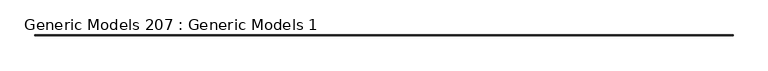
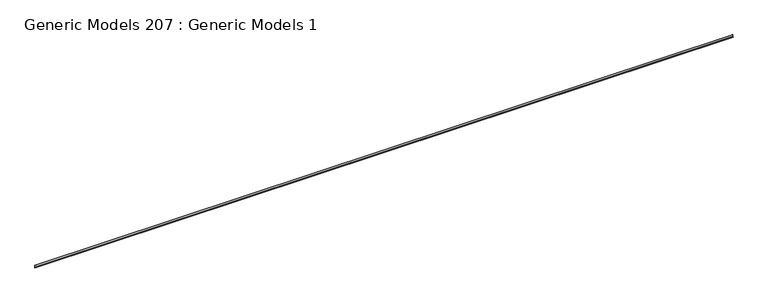
"""IFC4 building model written with IfcOpenShell, lengths in millimetres: proxy geometry, Generic Models 207 : Generic Models 1."""

import ifcopenshell
import ifcopenshell.guid

model = None  # the IFC model being written
_history = None  # IfcOwnerHistory: only IFC2X3 demands one
_inside = {}  # id of a spatial element -> (the spatial element, [elements in it])
_under = {}  # id of a project, library or spatial element -> (it, [spatial elements below it])
_declared = {}  # id of a project -> (the project, [libraries it declares])
_typed = {}  # id of a type object -> (the type object, [elements of that type])
_made_of = {}  # id of a material, layer set ... -> (it, [elements and type objects made of it])


def new_model(schema):
    """Start an empty IFC model of exactly this schema.

    Asked for "IFC4X3", IfcOpenShell would pick the latest addendum, in which some entities
    have other attributes; the version numbers below select the first issue.
    IFC2X3 requires an IfcOwnerHistory on every rooted entity: one is made here for all.
    """
    global model, _history
    if schema == "IFC4X3":
        model = ifcopenshell.file(schema_version=(4, 3, 0, 0))
    else:
        model = ifcopenshell.file(schema=schema)
    _inside.clear()
    _under.clear()
    _declared.clear()
    _typed.clear()
    _made_of.clear()
    _history = None
    if model.schema == "IFC2X3":
        org = make("IfcOrganization", Name="unknown")
        user = make(
            "IfcPersonAndOrganization",
            ThePerson=make("IfcPerson", FamilyName="unknown"),
            TheOrganization=org,
        )
        app = make(
            "IfcApplication",
            ApplicationDeveloper=org,
            Version="unknown",
            ApplicationFullName="unknown",
            ApplicationIdentifier="unknown",
        )
        _history = make(
            "IfcOwnerHistory",
            OwningUser=user,
            OwningApplication=app,
            ChangeAction="ADDED",
            CreationDate=0,
        )
    return model


def make(cls, **values):
    """One entity of the class cls with the attributes given. An attribute that is None is left unset."""
    return model.create_entity(
        cls, **{name: value for name, value in values.items() if value is not None}
    )


def rooted(cls, **values):
    """An entity with a GlobalId (a new one), such as an element, a storey or a relation."""
    return make(cls, GlobalId=ifcopenshell.guid.new(), OwnerHistory=_history, **values)


def si_unit(unit_type, name, prefix=None):
    """IfcSIUnit, for example si_unit("LENGTHUNIT", "METRE", prefix="MILLI")."""
    return make("IfcSIUnit", UnitType=unit_type, Prefix=prefix, Name=name)


def assignment(units):
    """IfcUnitAssignment: the units of a project."""
    return None if units is None else make("IfcUnitAssignment", Units=units)


def point(xyz):
    """IfcCartesianPoint."""
    return None if xyz is None else make("IfcCartesianPoint", Coordinates=xyz)


def direction(xyz):
    """IfcDirection."""
    return None if xyz is None else make("IfcDirection", DirectionRatios=xyz)


def frame(location, z_axis=None, x_axis=None):
    """IfcAxis2Placement3D, a coordinate frame: its origin and axes. An axis left out is left unset."""
    return make(
        "IfcAxis2Placement3D",
        Location=point(location),
        Axis=direction(z_axis),
        RefDirection=direction(x_axis),
    )


def origin():
    """The frame at (0, 0, 0) with its axes left unset."""
    return frame((0.0, 0.0, 0.0))


def place(relative_to, where):
    """IfcLocalPlacement: puts the frame where relative to a parent placement (None: the world)."""
    return make(
        "IfcLocalPlacement", PlacementRelTo=relative_to, RelativePlacement=where
    )


def context(
    kind, dimensions, precision=None, world=None, true_north=None, identifier=None
):
    """IfcGeometricRepresentationContext, for example the 3D "Model" context."""
    return make(
        "IfcGeometricRepresentationContext",
        ContextIdentifier=identifier,
        ContextType=kind,
        CoordinateSpaceDimension=dimensions,
        Precision=precision,
        WorldCoordinateSystem=world,
        TrueNorth=true_north,
    )


def project(units=None, contexts=None):
    """IfcProject with its units and contexts."""
    return rooted(
        "IfcProject",
        Name="project",
        RepresentationContexts=contexts,
        UnitsInContext=assignment(units),
    )


def spatial(cls, under=None, at=None, **own):
    """A site, building, storey or space (cls), placed at a placement, below another one or the project."""
    s = rooted(cls, ObjectPlacement=at, **own)
    if under is not None:
        _under.setdefault(under.id(), (under, []))[1].append(s)
    return s


def polyline(points):
    """IfcPolyline through the points."""
    return make("IfcPolyline", Points=[point(p) for p in points])


def outline(outer, holes=None, kind="AREA"):
    """IfcArbitraryClosedProfileDef: a profile drawn as a closed curve; with holes, ...WithVoids."""
    if holes is None:
        return make("IfcArbitraryClosedProfileDef", ProfileType=kind, OuterCurve=outer)
    return make(
        "IfcArbitraryProfileDefWithVoids",
        ProfileType=kind,
        OuterCurve=outer,
        InnerCurves=holes,
    )


def extrude(swept, where, along, depth):
    """IfcExtrudedAreaSolid: the profile swept, set in the frame where, extruded along a direction by depth."""
    return make(
        "IfcExtrudedAreaSolid",
        SweptArea=swept,
        Position=where,
        ExtrudedDirection=direction(along),
        Depth=depth,
    )


def shape(context_of_items, identifier, shape_type, items):
    """IfcShapeRepresentation: the items that make up one representation, for example the "Body"."""
    return make(
        "IfcShapeRepresentation",
        ContextOfItems=context_of_items,
        RepresentationIdentifier=identifier,
        RepresentationType=shape_type,
        Items=items,
    )


def source(mapping_origin, context_of_items, identifier, shape_type, items):
    """IfcRepresentationMap: a shape defined once, which mapped items show again and again."""
    return make(
        "IfcRepresentationMap",
        MappingOrigin=mapping_origin,
        MappedRepresentation=shape(context_of_items, identifier, shape_type, items),
    )


def transform(
    local_origin,
    x_axis=None,
    y_axis=None,
    z_axis=None,
    scale=None,
    scale2=None,
    scale3=None,
    uniform=True,
):
    """IfcCartesianTransformationOperator3D, or its non-uniform kind. x_axis, y_axis, z_axis: its Axis1, 2, 3."""
    if uniform:
        return make(
            "IfcCartesianTransformationOperator3D",
            Axis1=direction(x_axis),
            Axis2=direction(y_axis),
            LocalOrigin=point(local_origin),
            Scale=scale,
            Axis3=direction(z_axis),
        )
    return make(
        "IfcCartesianTransformationOperator3DnonUniform",
        Axis1=direction(x_axis),
        Axis2=direction(y_axis),
        LocalOrigin=point(local_origin),
        Scale=scale,
        Axis3=direction(z_axis),
        Scale2=scale2,
        Scale3=scale3,
    )


def mapped(mapping_source, mapping_target):
    """IfcMappedItem: shows the shape of a source again, moved by a transform."""
    return make(
        "IfcMappedItem", MappingSource=mapping_source, MappingTarget=mapping_target
    )


def made_of(thing, what):
    """Note that an element or type object is made of a material, layer set ...; save() writes the relation."""
    if what is not None:
        _made_of.setdefault(what.id(), (what, []))[1].append(thing)
    return thing


def element(
    cls,
    number,
    at=None,
    inside=None,
    cuts=None,
    type_object=None,
    material=None,
    context=None,
    identifier="Body",
    shape_type=None,
    held_by="IfcProductDefinitionShape",
    body=None,
    shapes=None,
    **own,
):
    """One element of the class cls, such as IfcWall. Its Tag is "e" and its number.

    at: its placement. inside: the storey or other place that contains it. cuts: it is an
    opening in that element (IfcRelVoidsElement). A single representation is given by context,
    identifier, shape_type and body (its items); several are given by shapes. held_by: the class
    of the entity that holds the representations. save() writes the other relations.
    """
    e = rooted(cls, Tag="e%d" % number, ObjectPlacement=at, **own)
    if body is not None:
        shapes = [shape(context, identifier, shape_type, body)]
    if shapes is not None:
        e.Representation = make(held_by, Representations=shapes)
    if inside is not None:
        _inside.setdefault(inside.id(), (inside, []))[1].append(e)
    if cuts is not None:
        rooted(
            "IfcRelVoidsElement", RelatingBuildingElement=cuts, RelatedOpeningElement=e
        )
    if type_object is not None:
        _typed.setdefault(type_object.id(), (type_object, []))[1].append(e)
    return made_of(e, material)


def aggregate(whole, parts):
    """IfcRelAggregates: a whole, such as a stair, and the parts it consists of."""
    return rooted("IfcRelAggregates", RelatingObject=whole, RelatedObjects=parts)


def save(model, path):
    """Write the relations noted so far, then the file.

    IfcRelAggregates (storeys below a building ...), IfcRelContainedInSpatialStructure (elements
    in a storey), IfcRelDefinesByType, IfcRelAssociatesMaterial and IfcRelDeclares: one each for
    every whole, place, type object, material and project.
    """
    for whole, parts in _under.values():
        aggregate(whole, parts)
    for where, things in _inside.values():
        rooted(
            "IfcRelContainedInSpatialStructure",
            RelatedElements=things,
            RelatingStructure=where,
        )
    for kind, things in _typed.values():
        rooted("IfcRelDefinesByType", RelatedObjects=things, RelatingType=kind)
    for what, things in _made_of.values():
        rooted("IfcRelAssociatesMaterial", RelatedObjects=things, RelatingMaterial=what)
    for by, libraries in _declared.values():
        rooted("IfcRelDeclares", RelatingContext=by, RelatedDefinitions=libraries)
    model.write(path)


def generic_models_207_generic_models_1_bd1820f3(model_context):
    return source(origin(), model_context, "Body", "SweptSolid", [
        extrude(outline(polyline([(6851.0769662, 123197.3823732), (6872.0319662, 123204.1179089), (6872.0319662, 123248.1823732), (6873.3019662, 123248.1823732), (6873.3019662, 123203.1921296), (6855.2271685, 123197.3823732), (6872.3387711, 123191.8822152), (6873.3019662, 123186.7674648), (6872.0539037, 123186.5324333), (6871.2305827, 123190.904425), (6851.0769662, 123197.3823732)])), frame((-10437.7171316, 0.0, 0.0), z_axis=(1.0, 0.0, 0.0), x_axis=(0.0, 1.0, 0.0)), (0.0, 0.0, 1.0), 19050.0),
    ])


if __name__ == "__main__":
    model = new_model("IFC4")
    model_context = context("Model", 3, world=origin())
    ifc_project = project(units=[si_unit("LENGTHUNIT", "METRE", prefix="MILLI")], contexts=[model_context])
    site = spatial("IfcSite", under=ifc_project)
    building = spatial("IfcBuilding", under=site)
    placement = place(None, origin())
    generic_models_207_generic_models_1_shape = generic_models_207_generic_models_1_bd1820f3(model_context)
    element("IfcBuildingElementProxy", 1, Name="Generic Models 207 : Generic Models 1", ObjectType="Generic Models 207 : Generic Models 1", at=placement, inside=building, context=model_context, shape_type="MappedRepresentation", body=[
        mapped(generic_models_207_generic_models_1_shape, transform((0.0, 0.0, 0.0), x_axis=(1.0, 0.0, 0.0), y_axis=(0.0, 1.0, 0.0), z_axis=(0.0, 0.0, 1.0))),
    ])
    save(model, "model.ifc")

# Revit data of these elements
# Element 1 (IfcBuildingElementProxy, "Generic Models 207 : Generic Models 1")
#   Materials on its faces: "_16 GA. COPPER WEEP SCREED W/ MIN. 3 1/2\" ATTACHEMENT FLANGE - LAP UNDERLAYMENT OVER WEED SCREED"
# Materials
#   "_16 GA. COPPER WEEP SCREED W/ MIN. 3 1/2\" ATTACHEMENT FLANGE - LAP UNDERLAYMENT OVER WEED SCREED": class "Generic", colour RGB 253 192 103, transparency 0, Cost = 0
